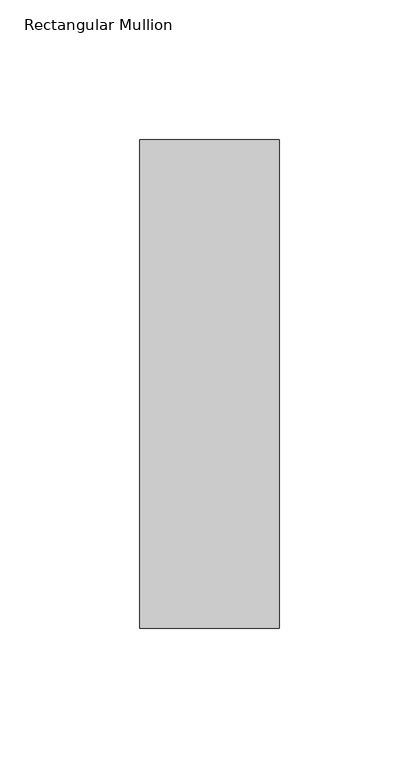
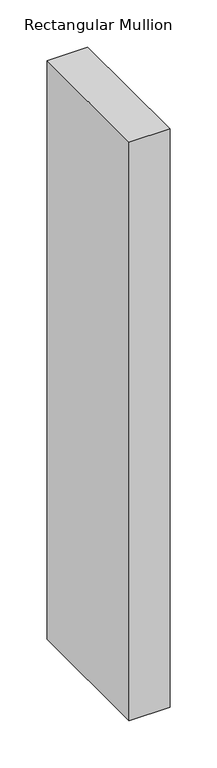
"""IFC4 building model written with IfcOpenShell, lengths in millimetres: member geometry, Rectangular Mullion : WWm-50x175-50mmOffset."""

import ifcopenshell
import ifcopenshell.guid

model = None  # the IFC model being written
_history = None  # IfcOwnerHistory: only IFC2X3 demands one
_inside = {}  # id of a spatial element -> (the spatial element, [elements in it])
_under = {}  # id of a project, library or spatial element -> (it, [spatial elements below it])
_declared = {}  # id of a project -> (the project, [libraries it declares])
_typed = {}  # id of a type object -> (the type object, [elements of that type])
_made_of = {}  # id of a material, layer set ... -> (it, [elements and type objects made of it])


def new_model(schema):
    """Start an empty IFC model of exactly this schema.

    Asked for "IFC4X3", IfcOpenShell would pick the latest addendum, in which some entities
    have other attributes; the version numbers below select the first issue.
    IFC2X3 requires an IfcOwnerHistory on every rooted entity: one is made here for all.
    """
    global model, _history
    if schema == "IFC4X3":
        model = ifcopenshell.file(schema_version=(4, 3, 0, 0))
    else:
        model = ifcopenshell.file(schema=schema)
    _inside.clear()
    _under.clear()
    _declared.clear()
    _typed.clear()
    _made_of.clear()
    _history = None
    if model.schema == "IFC2X3":
        org = make("IfcOrganization", Name="unknown")
        user = make(
            "IfcPersonAndOrganization",
            ThePerson=make("IfcPerson", FamilyName="unknown"),
            TheOrganization=org,
        )
        app = make(
            "IfcApplication",
            ApplicationDeveloper=org,
            Version="unknown",
            ApplicationFullName="unknown",
            ApplicationIdentifier="unknown",
        )
        _history = make(
            "IfcOwnerHistory",
            OwningUser=user,
            OwningApplication=app,
            ChangeAction="ADDED",
            CreationDate=0,
        )
    return model


def make(cls, **values):
    """One entity of the class cls with the attributes given. An attribute that is None is left unset."""
    return model.create_entity(
        cls, **{name: value for name, value in values.items() if value is not None}
    )


def rooted(cls, **values):
    """An entity with a GlobalId (a new one), such as an element, a storey or a relation."""
    return make(cls, GlobalId=ifcopenshell.guid.new(), OwnerHistory=_history, **values)


def si_unit(unit_type, name, prefix=None):
    """IfcSIUnit, for example si_unit("LENGTHUNIT", "METRE", prefix="MILLI")."""
    return make("IfcSIUnit", UnitType=unit_type, Prefix=prefix, Name=name)


def assignment(units):
    """IfcUnitAssignment: the units of a project."""
    return None if units is None else make("IfcUnitAssignment", Units=units)


def point(xyz):
    """IfcCartesianPoint."""
    return None if xyz is None else make("IfcCartesianPoint", Coordinates=xyz)


def direction(xyz):
    """IfcDirection."""
    return None if xyz is None else make("IfcDirection", DirectionRatios=xyz)


def frame(location, z_axis=None, x_axis=None):
    """IfcAxis2Placement3D, a coordinate frame: its origin and axes. An axis left out is left unset."""
    return make(
        "IfcAxis2Placement3D",
        Location=point(location),
        Axis=direction(z_axis),
        RefDirection=direction(x_axis),
    )


def origin():
    """The frame at (0, 0, 0) with its axes left unset."""
    return frame((0.0, 0.0, 0.0))


def place(relative_to, where):
    """IfcLocalPlacement: puts the frame where relative to a parent placement (None: the world)."""
    return make(
        "IfcLocalPlacement", PlacementRelTo=relative_to, RelativePlacement=where
    )


def context(
    kind, dimensions, precision=None, world=None, true_north=None, identifier=None
):
    """IfcGeometricRepresentationContext, for example the 3D "Model" context."""
    return make(
        "IfcGeometricRepresentationContext",
        ContextIdentifier=identifier,
        ContextType=kind,
        CoordinateSpaceDimension=dimensions,
        Precision=precision,
        WorldCoordinateSystem=world,
        TrueNorth=true_north,
    )


def project(units=None, contexts=None):
    """IfcProject with its units and contexts."""
    return rooted(
        "IfcProject",
        Name="project",
        RepresentationContexts=contexts,
        UnitsInContext=assignment(units),
    )


def spatial(cls, under=None, at=None, **own):
    """A site, building, storey or space (cls), placed at a placement, below another one or the project."""
    s = rooted(cls, ObjectPlacement=at, **own)
    if under is not None:
        _under.setdefault(under.id(), (under, []))[1].append(s)
    return s


def polyline(points):
    """IfcPolyline through the points."""
    return make("IfcPolyline", Points=[point(p) for p in points])


def outline(outer, holes=None, kind="AREA"):
    """IfcArbitraryClosedProfileDef: a profile drawn as a closed curve; with holes, ...WithVoids."""
    if holes is None:
        return make("IfcArbitraryClosedProfileDef", ProfileType=kind, OuterCurve=outer)
    return make(
        "IfcArbitraryProfileDefWithVoids",
        ProfileType=kind,
        OuterCurve=outer,
        InnerCurves=holes,
    )


def extrude(swept, where, along, depth):
    """IfcExtrudedAreaSolid: the profile swept, set in the frame where, extruded along a direction by depth."""
    return make(
        "IfcExtrudedAreaSolid",
        SweptArea=swept,
        Position=where,
        ExtrudedDirection=direction(along),
        Depth=depth,
    )


def shape(context_of_items, identifier, shape_type, items):
    """IfcShapeRepresentation: the items that make up one representation, for example the "Body"."""
    return make(
        "IfcShapeRepresentation",
        ContextOfItems=context_of_items,
        RepresentationIdentifier=identifier,
        RepresentationType=shape_type,
        Items=items,
    )


def source(mapping_origin, context_of_items, identifier, shape_type, items):
    """IfcRepresentationMap: a shape defined once, which mapped items show again and again."""
    return make(
        "IfcRepresentationMap",
        MappingOrigin=mapping_origin,
        MappedRepresentation=shape(context_of_items, identifier, shape_type, items),
    )


def transform(
    local_origin,
    x_axis=None,
    y_axis=None,
    z_axis=None,
    scale=None,
    scale2=None,
    scale3=None,
    uniform=True,
):
    """IfcCartesianTransformationOperator3D, or its non-uniform kind. x_axis, y_axis, z_axis: its Axis1, 2, 3."""
    if uniform:
        return make(
            "IfcCartesianTransformationOperator3D",
            Axis1=direction(x_axis),
            Axis2=direction(y_axis),
            LocalOrigin=point(local_origin),
            Scale=scale,
            Axis3=direction(z_axis),
        )
    return make(
        "IfcCartesianTransformationOperator3DnonUniform",
        Axis1=direction(x_axis),
        Axis2=direction(y_axis),
        LocalOrigin=point(local_origin),
        Scale=scale,
        Axis3=direction(z_axis),
        Scale2=scale2,
        Scale3=scale3,
    )


def mapped(mapping_source, mapping_target):
    """IfcMappedItem: shows the shape of a source again, moved by a transform."""
    return make(
        "IfcMappedItem", MappingSource=mapping_source, MappingTarget=mapping_target
    )


def made_of(thing, what):
    """Note that an element or type object is made of a material, layer set ...; save() writes the relation."""
    if what is not None:
        _made_of.setdefault(what.id(), (what, []))[1].append(thing)
    return thing


def element(
    cls,
    number,
    at=None,
    inside=None,
    cuts=None,
    type_object=None,
    material=None,
    context=None,
    identifier="Body",
    shape_type=None,
    held_by="IfcProductDefinitionShape",
    body=None,
    shapes=None,
    **own,
):
    """One element of the class cls, such as IfcWall. Its Tag is "e" and its number.

    at: its placement. inside: the storey or other place that contains it. cuts: it is an
    opening in that element (IfcRelVoidsElement). A single representation is given by context,
    identifier, shape_type and body (its items); several are given by shapes. held_by: the class
    of the entity that holds the representations. save() writes the other relations.
    """
    e = rooted(cls, Tag="e%d" % number, ObjectPlacement=at, **own)
    if body is not None:
        shapes = [shape(context, identifier, shape_type, body)]
    if shapes is not None:
        e.Representation = make(held_by, Representations=shapes)
    if inside is not None:
        _inside.setdefault(inside.id(), (inside, []))[1].append(e)
    if cuts is not None:
        rooted(
            "IfcRelVoidsElement", RelatingBuildingElement=cuts, RelatedOpeningElement=e
        )
    if type_object is not None:
        _typed.setdefault(type_object.id(), (type_object, []))[1].append(e)
    return made_of(e, material)


def aggregate(whole, parts):
    """IfcRelAggregates: a whole, such as a stair, and the parts it consists of."""
    return rooted("IfcRelAggregates", RelatingObject=whole, RelatedObjects=parts)


def save(model, path):
    """Write the relations noted so far, then the file.

    IfcRelAggregates (storeys below a building ...), IfcRelContainedInSpatialStructure (elements
    in a storey), IfcRelDefinesByType, IfcRelAssociatesMaterial and IfcRelDeclares: one each for
    every whole, place, type object, material and project.
    """
    for whole, parts in _under.values():
        aggregate(whole, parts)
    for where, things in _inside.values():
        rooted(
            "IfcRelContainedInSpatialStructure",
            RelatedElements=things,
            RelatingStructure=where,
        )
    for kind, things in _typed.values():
        rooted("IfcRelDefinesByType", RelatedObjects=things, RelatingType=kind)
    for what, things in _made_of.values():
        rooted("IfcRelAssociatesMaterial", RelatedObjects=things, RelatingMaterial=what)
    for by, libraries in _declared.values():
        rooted("IfcRelDeclares", RelatingContext=by, RelatedDefinitions=libraries)
    model.write(path)


def rectangular_mullion_73f72675(model_context):
    return source(origin(), model_context, "Body", "SweptSolid", [
        extrude(outline(polyline([(0.0, 87.5), (0.0, -87.5), (-50.0, -87.5), (-50.0, 87.5), (0.0, 87.5)])), frame((0.0, 0.0, -750.0), z_axis=(0.0, 0.0, 1.0), x_axis=(1.0, 0.0, 0.0)), (0.0, 0.0, 1.0), 750.0),
    ])


if __name__ == "__main__":
    model = new_model("IFC4")
    model_context = context("Model", 3, world=origin())
    ifc_project = project(units=[si_unit("LENGTHUNIT", "METRE", prefix="MILLI")], contexts=[model_context])
    site = spatial("IfcSite", under=ifc_project)
    building = spatial("IfcBuilding", under=site)
    placement = place(None, origin())
    rectangular_mullion_shape = rectangular_mullion_73f72675(model_context)
    element("IfcMember", 1, ObjectType="Rectangular Mullion : WWm-50x175-50mmOffset", at=placement, inside=building, context=model_context, shape_type="MappedRepresentation", body=[
        mapped(rectangular_mullion_shape, transform((0.0, 0.0, 0.0), x_axis=(1.0, 0.0, 0.0), y_axis=(0.0, 1.0, 0.0), z_axis=(0.0, 0.0, 1.0))),
    ])
    save(model, "model.ifc")

# Revit data of these elements
# Type "Rectangular Mullion : WWm-50x175-50mmOffset"
#   built-in parameter 1007304 = 0.574147 (stored number, unit not read)
#   built-in parameter 1007301 = 0.082021 (stored number, unit not read)
#   built-in parameter 1007300 = 0.082021 (stored number, unit not read)
# Element 1 (IfcMember, "Rectangular Mullion : WWm-50x175-50mmOffset")
#   Materials on its faces: "WW-EC-RGB-Mullion"
# Materials
#   "WW-EC-RGB-Mullion": class "Generic", colour RGB 255 255 255, transparency 0, Comments = "If region requests black mullions, switch asset color to RGB 25-25-25", Description = "Generic Color", Cost = 0
